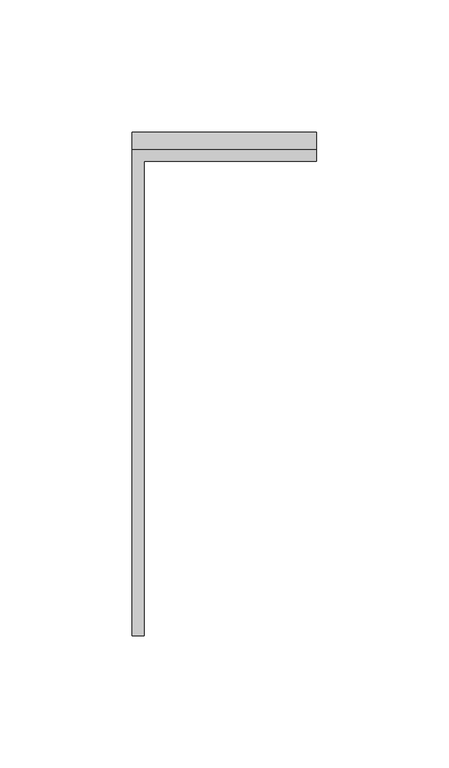
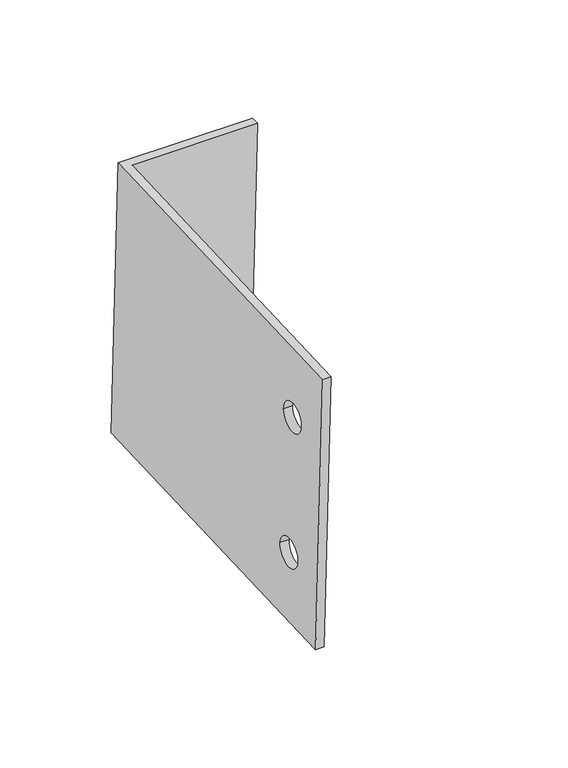
"""IFC4 building model written with IfcOpenShell, lengths in millimetres: proxy geometry, Generic Models 7:Generic Models 1:8:Generic Models 1:8 : Generic Models 7:Generic Models 1:337419:7 : Generic Models 7:Generic Models 1:8:Generic Models 1:8 : Generic Models 7:Generic Models 1:337419:315935."""

from ifc_helpers import new_model, si_unit, frame, origin, place, context, project, spatial, polyline, circle_curve, source, transform, mapped, element, save
from ifc_brep_helpers import plane_surface, revolved_surface, advanced_brep


def generic_models_e83c5f3e(model_context):
    return source(origin(), model_context, "Body", "AdvancedBrep", [
        advanced_brep(
        [(593804.563286, -564939.7244578, 8729.2523376), (593804.563286, -564760.2942082, 8736.728598), (593804.563286, -564766.6387032, 8888.9964783), (593804.563286, -564946.0689528, 8881.5202179), (593804.563286, -564911.167349, 8844.5106637), (593804.563286, -564927.042349, 8844.5106637), (593804.563286, -564908.0226145, 8769.0370354), (593804.563286, -564923.8425885, 8767.7164115), (593799.9992235, -564946.0689528, 8881.5202179), (593799.9992235, -564939.7244578, 8729.2523376), (593799.9992235, -564911.167349, 8844.5106637), (593799.9992235, -564927.042349, 8844.5106637), (593799.9992235, -564908.0226145, 8769.0370354), (593799.9992235, -564923.8425885, 8767.7164115), (593869.8492235, -564755.7341024, 8736.9186024), (593799.9992235, -564755.7341024, 8736.9186024), (593799.9992235, -564762.0785974, 8889.1864827), (593869.8492235, -564762.0785974, 8889.1864827), (593869.8492235, -564760.2942082, 8736.728598), (593869.8492235, -564766.6387032, 8888.9964783)],
        [
            (0, 1),
            (1, 2),
            (2, 3),
            (3, 0),
            (4, 5, circle_curve(frame((593804.563286, -564919.104849, 8844.5106637), z_axis=(-1.0, 0.0, 0.0), x_axis=(0.0, -1.0, 0.0)), 7.9375)),
            (5, 4, circle_curve(frame((593804.563286, -564919.104849, 8844.5106637), z_axis=(-1.0, 0.0, 0.0), x_axis=(0.0, -1.0, 0.0)), 7.9375)),
            (6, 7, circle_curve(frame((593804.563286, -564915.9326015, 8768.3767235), z_axis=(-1.0, 0.0, 0.0), x_axis=(0.0, -0.9965337954939333, -0.08318890814559193)), 7.9375)),
            (7, 6, circle_curve(frame((593804.563286, -564915.9326015, 8768.3767235), z_axis=(-1.0, 0.0, 0.0), x_axis=(0.0, -0.9965337954939333, -0.08318890814559193)), 7.9375)),
            (3, 8),
            (8, 9),
            (9, 0),
            (4, 10),
            (10, 11, circle_curve(frame((593799.9992235, -564919.104849, 8844.5106637), z_axis=(-1.0, 0.0, 0.0), x_axis=(0.0, -1.0, 0.0)), 7.9375)),
            (11, 5),
            (11, 10, circle_curve(frame((593799.9992235, -564919.104849, 8844.5106637), z_axis=(-1.0, 0.0, 0.0), x_axis=(0.0, -1.0, 0.0)), 7.9375)),
            (6, 12),
            (12, 13, circle_curve(frame((593799.9992235, -564915.9326015, 8768.3767235), z_axis=(-1.0, 0.0, 0.0), x_axis=(0.0, -0.9965337954939333, -0.08318890814559193)), 7.9375)),
            (13, 7),
            (13, 12, circle_curve(frame((593799.9992235, -564915.9326015, 8768.3767235), z_axis=(-1.0, 0.0, 0.0), x_axis=(0.0, -0.9965337954939333, -0.08318890814559193)), 7.9375)),
            (14, 15),
            (15, 16),
            (16, 17),
            (17, 14),
            (18, 19),
            (19, 2),
            (1, 18),
            (17, 19),
            (18, 14),
            (9, 15),
            (8, 16),
        ],
        [
            plane_surface(frame((593804.563286, -564938.7460392, 8705.7702907), z_axis=(1.0, 0.0, 0.0), x_axis=(0.0, 0.04163054470882304, -0.9991330730924919))),
            plane_surface(frame((593799.9992235, -564939.7244578, 8729.2523376), z_axis=(0.0, -0.9991330730924919, -0.04163054470882304), x_axis=(1.0, 0.0, 0.0))),
            revolved_surface(polyline([(593804.563286, -564927.042349, 8844.5106637), (593799.9992235, -564927.042349, 8844.5106637)]), (598681.363286, -564919.104849, 8844.5106637), (1.0, 0.0, 0.0)),
            revolved_surface(polyline([(593804.563286, -564923.8425885016, 8767.716411541594), (593799.9992235, -564923.8425885016, 8767.716411541594)]), (598681.363286, -564915.9326015, 8768.3767235), (1.0000000000000002, 0.0, 0.0)),
            plane_surface(frame((593869.8492235, -564754.7556838, 8713.4365555), z_axis=(4.4453795977400165e-12, 0.9991330730923519, 0.041630544712183803), x_axis=(3.637978807094492e-12, 0.041630544712183803, -0.9991330730923519))),
            plane_surface(frame((593869.8492235, -564759.3157896, 8713.2465511), z_axis=(-4.4453795977400165e-12, -0.9991330730923519, -0.041630544712183803), x_axis=(-3.637978807094492e-12, -0.041630544712183803, 0.9991330730923519))),
            plane_surface(frame((593869.8492235, -564760.2942082, 8736.728598), z_axis=(1.0, 0.0, 3.634824945374345e-12), x_axis=(0.0, 0.9991330730923487, 0.04163054471226028))),
            plane_surface(frame((593799.9992235, -564760.2942082, 8736.728598), z_axis=(0.0, 0.04163054471226028, -0.9991330730923487), x_axis=(0.0, 0.9991330730923487, 0.04163054471226028))),
            plane_surface(frame((593799.9992235, -564766.6387032, 8888.9964783), z_axis=(-1.0, 0.0, 0.0), x_axis=(0.0, 0.9991330730923487, 0.04163054471226028))),
            plane_surface(frame((593869.8492235, -564766.6387032, 8888.9964783), z_axis=(0.0, -0.04163054471202344, 0.9991330730923585), x_axis=(0.0, 0.9991330730923585, 0.04163054471202344))),
        ],
        [
            (0, [[1, 2, 3, 4], [5, 6], [7, 8]]),
            (1, [[-4, 9, 10, 11]]),
            (2, [[-5, 12, 13, 14]]),
            (2, [[-6, -14, 15, -12]]),
            (3, [[-7, 16, 17, 18]]),
            (3, [[-8, -18, 19, -16]]),
            (4, [[20, 21, 22, 23]]),
            (5, [[24, 25, -2, 26]]),
            (6, [[-23, 27, -24, 28]]),
            (7, [[-20, -28, -26, -1, -11, 29]]),
            (8, [[-21, -29, -10, 30], [-15, -13], [-19, -17]]),
            (9, [[-22, -30, -9, -3, -25, -27]]),
        ],
    ),
    ])


if __name__ == "__main__":
    model = new_model("IFC4")
    model_context = context("Model", 3, world=origin())
    ifc_project = project(units=[si_unit("LENGTHUNIT", "METRE", prefix="MILLI")], contexts=[model_context])
    site = spatial("IfcSite", under=ifc_project)
    building = spatial("IfcBuilding", under=site)
    placement = place(None, origin())
    generic_models_shape = generic_models_e83c5f3e(model_context)
    element("IfcBuildingElementProxy", 1, Name="Generic Models 7:Generic Models 1:8:Generic Models 1:8 : Generic Models 7:Generic Models 1:337419:7 : Generic Models 7:Generic Models 1:8:Generic Models 1:8 : Generic Models 7:Generic Models 1:337419:315935", ObjectType="Generic Models 7:Generic Models 1:8:Generic Models 1:8 : Generic Models 7:Generic Models 1:337419:7 : Generic Models 7:Generic Models 1:8:Generic Models 1:8 : Generic Models 7:Generic Models 1:337419:315935", at=placement, inside=building, context=model_context, shape_type="MappedRepresentation", body=[
        mapped(generic_models_shape, transform((0.0, 0.0, 0.0), x_axis=(1.0, 0.0, 0.0), y_axis=(0.0, 1.0, 0.0), z_axis=(0.0, 0.0, 1.0))),
    ])
    save(model, "model.ifc")

# Revit data of these elements
# Type "Generic Models 7:Generic Models 1:8:Generic Models 1:8 : Generic Models 7:Generic Models 1:337419:7 : Generic Models 7:Generic Models 1:8:Generic Models 1:8 : Generic Models 7:Generic Models 1:337419:315935"
#   NameOverride = "Generic Models 7:Generic Models 1:8:Generic Models 1:8 : Generic Models 7:Generic Models 1:337419:315935"
#   ObjectTypeOverride = "Generic Models 1:8 : Generic Models 7:Generic Models 1:337419"
#   Reference = "Generic Models 1"
#   Tag = "315935"
# Element 1 (IfcBuildingElementProxy, "Generic Models 7:Generic Models 1:8:Generic Models 1:8 : Generic Models 7:Generic Models 1:337419:7 : Generic Models 7:Generic Models 1:8:Generic Models 1:8 : Generic Models 7:Generic Models 1:337419:315935")
#   Materials on its faces: "0.179\" THICK BENT STEEL CLIPS"
# Materials
#   "0.179\" THICK BENT STEEL CLIPS": class "Metal", colour RGB 189 187 185, transparency 0, Description = "Structural steel 50ksi", Cost = 0
